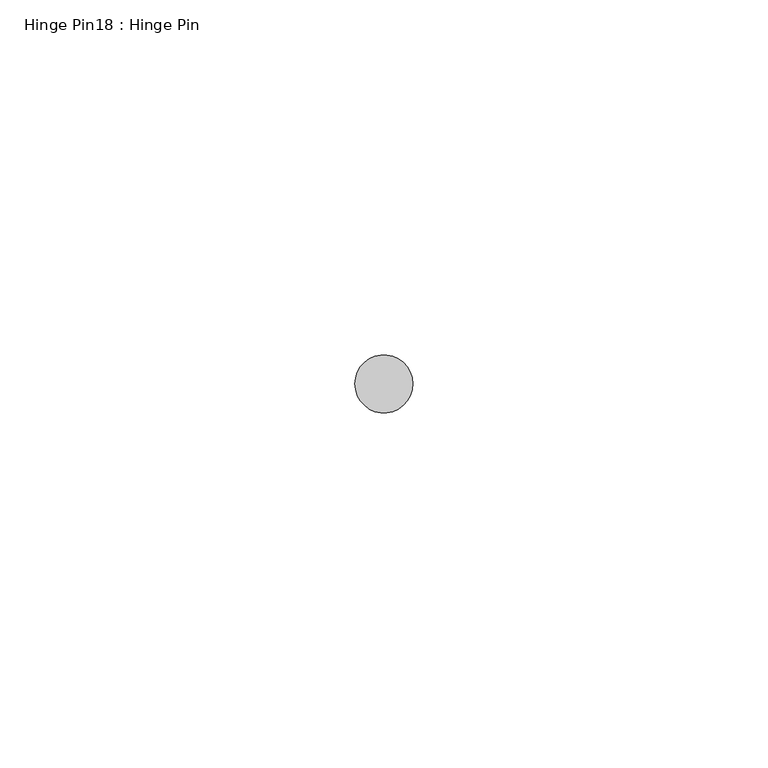
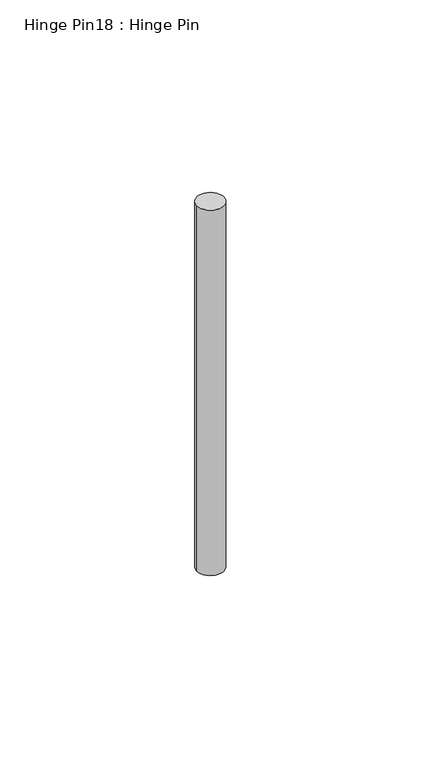
"""IFC4 building model written with IfcOpenShell, lengths in millimetres: proxy geometry, Hinge Pin18 : Hinge Pin."""

from ifc_helpers import new_model, si_unit, point, frame, frame_2d, origin, place, context, project, spatial, circle_curve, trimmed, segment, composite_curve, outline, extrude, source, transform, mapped, element, save


def hinge_pin18_hinge_pin_e1ebbe44(model_context):
    return source(origin(), model_context, "Body", "SweptSolid", [
        extrude(outline(composite_curve([segment(trimmed(circle_curve(frame_2d((587319.1320739, -534100.7049841)), 4.0894), [point((587315.0426739, -534100.7049841))], [point((587323.2214739, -534100.7049841))], False, "CARTESIAN"), True, "CONTINUOUS"), segment(trimmed(circle_curve(frame_2d((587319.1320739, -534100.7049841)), 4.0894), [point((587323.2214739, -534100.7049841))], [point((587315.0426739, -534100.7049841))], False, "CARTESIAN"), True, "CONTINUOUS")], self_intersect=False)), frame((0.0, 0.0, 315.7140625), z_axis=(0.0, 0.0, 1.0), x_axis=(1.0, 0.0, 0.0)), (0.0, 0.0, 1.0), 117.871875),
    ])


if __name__ == "__main__":
    model = new_model("IFC4")
    model_context = context("Model", 3, world=origin())
    ifc_project = project(units=[si_unit("LENGTHUNIT", "METRE", prefix="MILLI")], contexts=[model_context])
    site = spatial("IfcSite", under=ifc_project)
    building = spatial("IfcBuilding", under=site)
    placement = place(None, origin())
    hinge_pin18_hinge_pin_shape = hinge_pin18_hinge_pin_e1ebbe44(model_context)
    element("IfcBuildingElementProxy", 1, Name="Hinge Pin18 : Hinge Pin", ObjectType="Hinge Pin18 : Hinge Pin", at=placement, inside=building, context=model_context, shape_type="MappedRepresentation", body=[
        mapped(hinge_pin18_hinge_pin_shape, transform((0.0, 0.0, 0.0), x_axis=(1.0, 0.0, 0.0), y_axis=(0.0, 1.0, 0.0), z_axis=(0.0, 0.0, 1.0))),
    ])
    save(model, "model.ifc")

# Revit data of these elements
# Element 1 (IfcBuildingElementProxy, "Hinge Pin18 : Hinge Pin")
#   Materials on its faces: "6\"X6\" WELD-ON STL BUTT HINGE"
# Materials
#   "6\"X6\" WELD-ON STL BUTT HINGE": class "Metal", colour RGB 189 187 185, transparency 0, Description = "Carbon steel", Cost = 0
